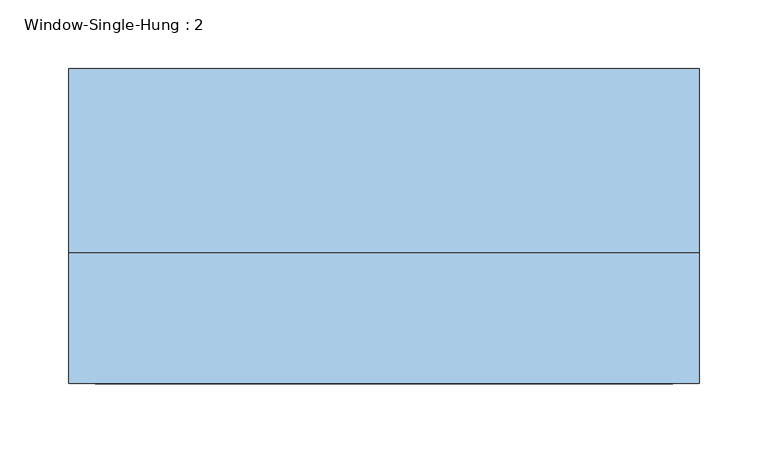
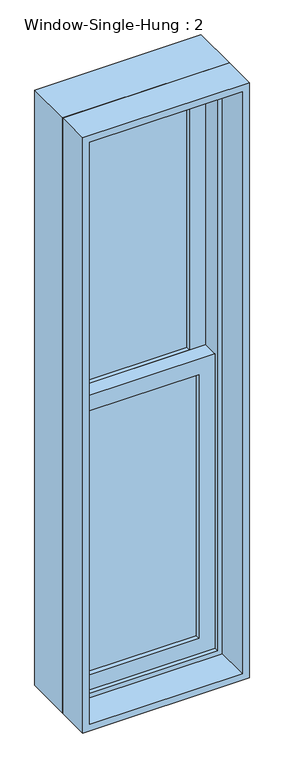
"""IFC4 building model written with IfcOpenShell, lengths in millimetres: window geometry, Window-Single-Hung : 2."""

from ifc_helpers import new_model, si_unit, frame, origin, place, context, project, spatial, polyline, outline, extrude, source, transform, mapped, element, save


def window_single_hung_2_a24a598a(model_context):
    return source(origin(), model_context, "Body", "SweptSolid", [
        extrude(outline(polyline([(152.4, 34.925), (152.4, 28.575), (-152.4, 28.575), (-152.4, 34.925), (152.4, 34.925)])), frame((0.0, 0.0, 990.6), z_axis=(0.0, 0.0, 1.0), x_axis=(1.0, 0.0, 0.0)), (0.0, 0.0, 1.0), 765.175),
        extrude(outline(polyline([(-152.4, 22.225), (152.4, 22.225), (152.4, 15.875), (-152.4, 15.875), (-152.4, 22.225)])), frame((0.0, 0.0, 990.6), z_axis=(0.0, 0.0, 1.0), x_axis=(1.0, 0.0, 0.0)), (0.0, 0.0, 1.0), 765.175),
        extrude(outline(polyline([(152.4, 79.375), (152.4, 73.025), (-152.4, 73.025), (-152.4, 79.375), (152.4, 79.375)])), frame((0.0, 0.0, 1800.225), z_axis=(0.0, 0.0, 1.0), x_axis=(1.0, 0.0, 0.0)), (0.0, 0.0, 1.0), 765.175),
        extrude(outline(polyline([(-152.4, 66.675), (152.4, 66.675), (152.4, 60.325), (-152.4, 60.325), (-152.4, 66.675)])), frame((0.0, 0.0, 1800.225), z_axis=(0.0, 0.0, 1.0), x_axis=(1.0, 0.0, 0.0)), (0.0, 0.0, 1.0), 765.175),
        extrude(outline(polyline([(1800.225, -196.85), (946.15, -196.85), (946.15, 196.85), (1800.225, 196.85), (1800.225, -196.85)]), holes=[polyline([(1755.775, 152.4), (990.6, 152.4), (990.6, -152.4), (1755.775, -152.4), (1755.775, 152.4)])]), frame((0.0, 3.175, 0.0), z_axis=(0.0, 1.0, 0.0), x_axis=(0.0, 0.0, 1.0)), (0.0, 0.0, 1.0), 44.45),
        extrude(outline(polyline([(2609.85, -196.85), (1755.775, -196.85), (1755.775, 196.85), (2609.85, 196.85), (2609.85, -196.85)]), holes=[polyline([(2565.4, 152.4), (1800.225, 152.4), (1800.225, -152.4), (2565.4, -152.4), (2565.4, 152.4)])]), frame((0.0, 47.625, 0.0), z_axis=(0.0, 1.0, 0.0), x_axis=(0.0, 0.0, 1.0)), (0.0, 0.0, 1.0), 44.45),
        extrude(outline(polyline([(2641.6, -228.6), (914.4, -228.6), (914.4, 228.6), (2641.6, 228.6), (2641.6, -228.6)]), holes=[polyline([(2609.85, 196.85), (946.15, 196.85), (946.15, -196.85), (2609.85, -196.85), (2609.85, 196.85)])]), frame((0.0, -9.525, 0.0), z_axis=(0.0, 1.0, 0.0), x_axis=(0.0, 0.0, 1.0)), (0.0, 0.0, 1.0), 133.35),
        extrude(outline(polyline([(2641.6, 228.6), (2641.6, -228.6), (914.4, -228.6), (914.4, 228.6), (2641.6, 228.6)]), holes=[polyline([(2622.55, 209.55), (933.45, 209.55), (933.45, -209.55), (2622.55, -209.55), (2622.55, 209.55)])]), frame((0.0, -104.775, 0.0), z_axis=(0.0, 1.0, 0.0), x_axis=(0.0, 0.0, 1.0)), (0.0, 0.0, 1.0), 95.25),
    ])


if __name__ == "__main__":
    model = new_model("IFC4")
    model_context = context("Model", 3, world=origin())
    ifc_project = project(units=[si_unit("LENGTHUNIT", "METRE", prefix="MILLI")], contexts=[model_context])
    site = spatial("IfcSite", under=ifc_project)
    building = spatial("IfcBuilding", under=site)
    placement = place(None, origin())
    window_single_hung_2_shape = window_single_hung_2_a24a598a(model_context)
    element("IfcWindow", 1, ObjectType="Window-Single-Hung : 2", at=placement, inside=building, context=model_context, shape_type="MappedRepresentation", body=[
        mapped(window_single_hung_2_shape, transform((0.0, 0.0, 0.0), x_axis=(1.0, 0.0, 0.0), y_axis=(0.0, 1.0, 0.0), z_axis=(0.0, 0.0, 1.0))),
    ])
    save(model, "model.ifc")

# Revit data of these elements
# Type "Window-Single-Hung : 2"
#   Type Mark = "13"
#   Fire Rating = "0.5h"
#   Construction Type Id = "DG-DR"
#   Assembly Code = "B2020100"
#   Analytic Construction = "Double glazing - domestic"
#   Wall Thickness [instance default] = 0' - 6"
#   Window Inset [instance default] = 0' - 0"
#   Visual Light Transmittance = 0.81
#   Thermal Resistance (R) = 0.319569 (m²·K)/W
#   Solar Heat Gain Coefficient = 0.76
#   Muntin Width = 1' - 0"
#   Muntin Height = 2' - 6 1/8"
#   Interior Wall Closure [instance default] = 0' - 1 1/2"
#   Rough Width = 1' - 6 1/2"
#   Rough Height = 5' - 8 1/2"
#   Frame Extension [instance default] = 0' - 1 1/4"
#   Exterior Wall Closure [instance default] = 0' - 0 1/2"
#   Extension Jamb [instance default] = 0' - 1 1/2"
#   Heat Transfer Coefficient (U) = 3.12929 W/(m²·K)
#   Height = 5' - 8"
#   Width = 1' - 6"
#   Top Muntin Visibility = yes
#   Indicator Visibility = no
#   Extension Jamb Visibility [instance default] = yes
#   Interior Trim Visibility [instance default] = yes
#   Exterior Trim Visibility [instance default] = yes
#   Bottom Muntin Visibility = no
#   Muntin Pattern = Muntin Pattern_2x2 : Muntin Pattern_2x2
#   Interior Trim Material = 1X WOOD COMPOSITE TRIM
#   Interior Trim = Trim-Window-Interior-Flat : Picture Frame
#   Exterior Trim Material = 1X WOOD COMPOSITE TRIM
#   Exterior Trim = Trim-Window-Exterior-Flat : with Sill
#   Glass Panel Material = NEW DOUBLE HUNG WINDOWS (TYP.)
#   Exterior Frame Material = 1X WOOD COMPOSITE TRIM
#   Interior Frame Material = 1X WOOD COMPOSITE TRIM
#   Wall Closure = (empty or 0)
# Element 1 (IfcWindow, "Window-Single-Hung : 2")
#   Wall Thickness = 0' - 8 1/4"
#   Extension Jamb = 0' - 3 3/4"
#   Materials on its faces: "1X WOOD COMPOSITE TRIM", "NEW DOUBLE HUNG WINDOWS (TYP.)"
# Materials
#   "1X WOOD COMPOSITE TRIM": class "Generic", colour RGB 88 61 61, transparency 0, Cost = 0
#   "NEW DOUBLE HUNG WINDOWS (TYP.)": class "Glass", colour RGB 218 227 224, transparency 0.85, Description = "Soda Lime Glass", Cost = 0
